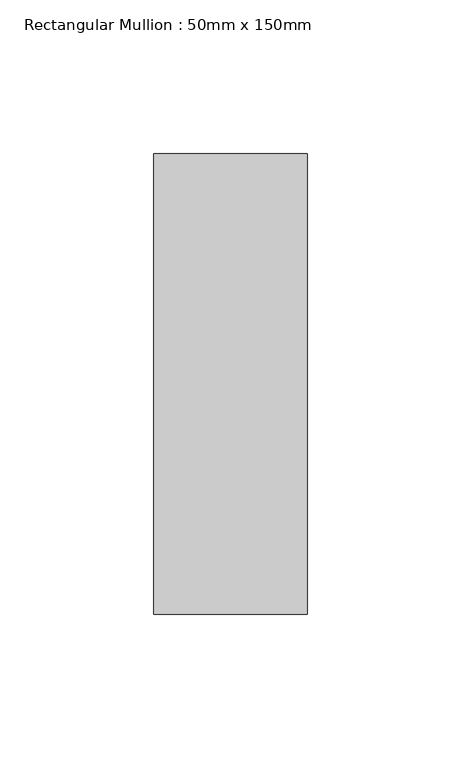
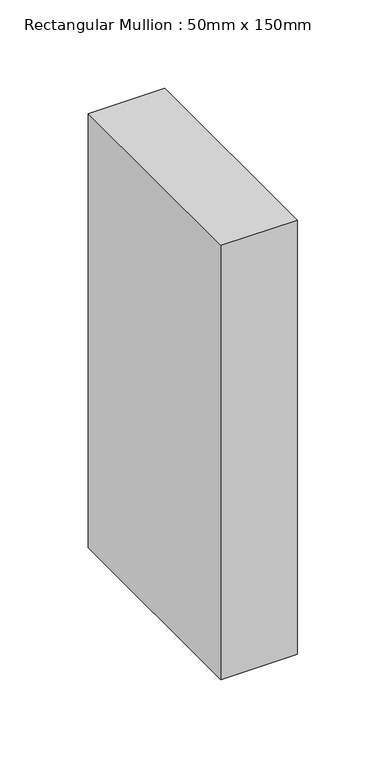
"""IFC4 building model written with IfcOpenShell, lengths in millimetres: member geometry, Rectangular Mullion : 50mm x 150mm."""

from ifc_helpers import new_model, si_unit, frame, origin, place, context, project, spatial, polyline, outline, extrude, source, transform, mapped, element, save


def rectangular_mullion_50mm_x_150mm_82697a32(model_context):
    return source(origin(), model_context, "Body", "SweptSolid", [
        extrude(outline(polyline([(0.0, 75.0), (0.0, -75.0), (-50.0, -75.0), (-50.0, 75.0), (0.0, 75.0)])), frame((0.0, 0.0, -300.0), z_axis=(0.0, 0.0, 1.0), x_axis=(1.0, 0.0, 0.0)), (0.0, 0.0, 1.0), 300.0),
    ])


if __name__ == "__main__":
    model = new_model("IFC4")
    model_context = context("Model", 3, world=origin())
    ifc_project = project(units=[si_unit("LENGTHUNIT", "METRE", prefix="MILLI")], contexts=[model_context])
    site = spatial("IfcSite", under=ifc_project)
    building = spatial("IfcBuilding", under=site)
    placement = place(None, origin())
    rectangular_mullion_50mm_x_150mm_shape = rectangular_mullion_50mm_x_150mm_82697a32(model_context)
    element("IfcMember", 1, ObjectType="Rectangular Mullion : 50mm x 150mm", at=placement, inside=building, context=model_context, shape_type="MappedRepresentation", body=[
        mapped(rectangular_mullion_50mm_x_150mm_shape, transform((0.0, 0.0, 0.0), x_axis=(1.0, 0.0, 0.0), y_axis=(0.0, 1.0, 0.0), z_axis=(0.0, 0.0, 1.0))),
    ])
    save(model, "model.ifc")

# Revit data of these elements
# Type "Rectangular Mullion : 50mm x 150mm"
#   built-in parameter 1007304 = 0.492126 (stored number, unit not read)
#   built-in parameter 1007301 = 0.082021 (stored number, unit not read)
#   built-in parameter 1007300 = 0.082021 (stored number, unit not read)
# Element 1 (IfcMember, "Rectangular Mullion : 50mm x 150mm")
#   Materials on its faces: "Aluminum"
# Materials
#   "Aluminum": class "Metal", colour RGB 244 244 244, transparency 0, Description = "Aluminum 6061", Cost = 0
